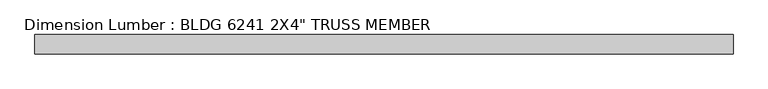
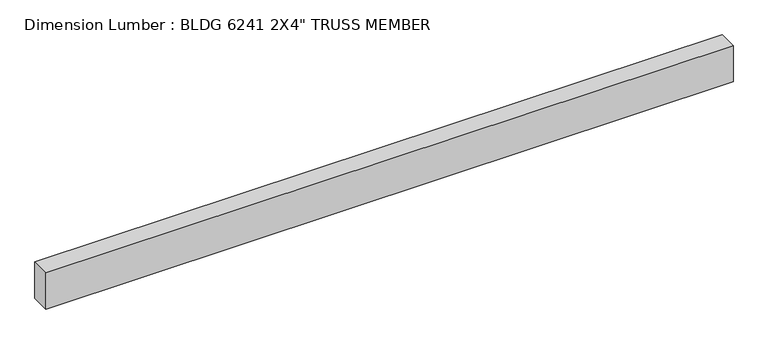
"""IFC4 building model written with IfcOpenShell, lengths in millimetres: beam geometry."""

import ifcopenshell
import ifcopenshell.guid

model = None  # the IFC model being written
_history = None  # IfcOwnerHistory: only IFC2X3 demands one
_inside = {}  # id of a spatial element -> (the spatial element, [elements in it])
_under = {}  # id of a project, library or spatial element -> (it, [spatial elements below it])
_declared = {}  # id of a project -> (the project, [libraries it declares])
_typed = {}  # id of a type object -> (the type object, [elements of that type])
_made_of = {}  # id of a material, layer set ... -> (it, [elements and type objects made of it])


def new_model(schema):
    """Start an empty IFC model of exactly this schema.

    Asked for "IFC4X3", IfcOpenShell would pick the latest addendum, in which some entities
    have other attributes; the version numbers below select the first issue.
    IFC2X3 requires an IfcOwnerHistory on every rooted entity: one is made here for all.
    """
    global model, _history
    if schema == "IFC4X3":
        model = ifcopenshell.file(schema_version=(4, 3, 0, 0))
    else:
        model = ifcopenshell.file(schema=schema)
    _inside.clear()
    _under.clear()
    _declared.clear()
    _typed.clear()
    _made_of.clear()
    _history = None
    if model.schema == "IFC2X3":
        org = make("IfcOrganization", Name="unknown")
        user = make(
            "IfcPersonAndOrganization",
            ThePerson=make("IfcPerson", FamilyName="unknown"),
            TheOrganization=org,
        )
        app = make(
            "IfcApplication",
            ApplicationDeveloper=org,
            Version="unknown",
            ApplicationFullName="unknown",
            ApplicationIdentifier="unknown",
        )
        _history = make(
            "IfcOwnerHistory",
            OwningUser=user,
            OwningApplication=app,
            ChangeAction="ADDED",
            CreationDate=0,
        )
    return model


def make(cls, **values):
    """One entity of the class cls with the attributes given. An attribute that is None is left unset."""
    return model.create_entity(
        cls, **{name: value for name, value in values.items() if value is not None}
    )


def rooted(cls, **values):
    """An entity with a GlobalId (a new one), such as an element, a storey or a relation."""
    return make(cls, GlobalId=ifcopenshell.guid.new(), OwnerHistory=_history, **values)


def si_unit(unit_type, name, prefix=None):
    """IfcSIUnit, for example si_unit("LENGTHUNIT", "METRE", prefix="MILLI")."""
    return make("IfcSIUnit", UnitType=unit_type, Prefix=prefix, Name=name)


def assignment(units):
    """IfcUnitAssignment: the units of a project."""
    return None if units is None else make("IfcUnitAssignment", Units=units)


def point(xyz):
    """IfcCartesianPoint."""
    return None if xyz is None else make("IfcCartesianPoint", Coordinates=xyz)


def direction(xyz):
    """IfcDirection."""
    return None if xyz is None else make("IfcDirection", DirectionRatios=xyz)


def frame(location, z_axis=None, x_axis=None):
    """IfcAxis2Placement3D, a coordinate frame: its origin and axes. An axis left out is left unset."""
    return make(
        "IfcAxis2Placement3D",
        Location=point(location),
        Axis=direction(z_axis),
        RefDirection=direction(x_axis),
    )


def origin():
    """The frame at (0, 0, 0) with its axes left unset."""
    return frame((0.0, 0.0, 0.0))


def place(relative_to, where):
    """IfcLocalPlacement: puts the frame where relative to a parent placement (None: the world)."""
    return make(
        "IfcLocalPlacement", PlacementRelTo=relative_to, RelativePlacement=where
    )


def context(
    kind, dimensions, precision=None, world=None, true_north=None, identifier=None
):
    """IfcGeometricRepresentationContext, for example the 3D "Model" context."""
    return make(
        "IfcGeometricRepresentationContext",
        ContextIdentifier=identifier,
        ContextType=kind,
        CoordinateSpaceDimension=dimensions,
        Precision=precision,
        WorldCoordinateSystem=world,
        TrueNorth=true_north,
    )


def project(units=None, contexts=None):
    """IfcProject with its units and contexts."""
    return rooted(
        "IfcProject",
        Name="project",
        RepresentationContexts=contexts,
        UnitsInContext=assignment(units),
    )


def spatial(cls, under=None, at=None, **own):
    """A site, building, storey or space (cls), placed at a placement, below another one or the project."""
    s = rooted(cls, ObjectPlacement=at, **own)
    if under is not None:
        _under.setdefault(under.id(), (under, []))[1].append(s)
    return s


def polyline(points):
    """IfcPolyline through the points."""
    return make("IfcPolyline", Points=[point(p) for p in points])


def outline(outer, holes=None, kind="AREA"):
    """IfcArbitraryClosedProfileDef: a profile drawn as a closed curve; with holes, ...WithVoids."""
    if holes is None:
        return make("IfcArbitraryClosedProfileDef", ProfileType=kind, OuterCurve=outer)
    return make(
        "IfcArbitraryProfileDefWithVoids",
        ProfileType=kind,
        OuterCurve=outer,
        InnerCurves=holes,
    )


def extrude(swept, where, along, depth):
    """IfcExtrudedAreaSolid: the profile swept, set in the frame where, extruded along a direction by depth."""
    return make(
        "IfcExtrudedAreaSolid",
        SweptArea=swept,
        Position=where,
        ExtrudedDirection=direction(along),
        Depth=depth,
    )


def shape(context_of_items, identifier, shape_type, items):
    """IfcShapeRepresentation: the items that make up one representation, for example the "Body"."""
    return make(
        "IfcShapeRepresentation",
        ContextOfItems=context_of_items,
        RepresentationIdentifier=identifier,
        RepresentationType=shape_type,
        Items=items,
    )


def source(mapping_origin, context_of_items, identifier, shape_type, items):
    """IfcRepresentationMap: a shape defined once, which mapped items show again and again."""
    return make(
        "IfcRepresentationMap",
        MappingOrigin=mapping_origin,
        MappedRepresentation=shape(context_of_items, identifier, shape_type, items),
    )


def transform(
    local_origin,
    x_axis=None,
    y_axis=None,
    z_axis=None,
    scale=None,
    scale2=None,
    scale3=None,
    uniform=True,
):
    """IfcCartesianTransformationOperator3D, or its non-uniform kind. x_axis, y_axis, z_axis: its Axis1, 2, 3."""
    if uniform:
        return make(
            "IfcCartesianTransformationOperator3D",
            Axis1=direction(x_axis),
            Axis2=direction(y_axis),
            LocalOrigin=point(local_origin),
            Scale=scale,
            Axis3=direction(z_axis),
        )
    return make(
        "IfcCartesianTransformationOperator3DnonUniform",
        Axis1=direction(x_axis),
        Axis2=direction(y_axis),
        LocalOrigin=point(local_origin),
        Scale=scale,
        Axis3=direction(z_axis),
        Scale2=scale2,
        Scale3=scale3,
    )


def mapped(mapping_source, mapping_target):
    """IfcMappedItem: shows the shape of a source again, moved by a transform."""
    return make(
        "IfcMappedItem", MappingSource=mapping_source, MappingTarget=mapping_target
    )


def made_of(thing, what):
    """Note that an element or type object is made of a material, layer set ...; save() writes the relation."""
    if what is not None:
        _made_of.setdefault(what.id(), (what, []))[1].append(thing)
    return thing


def element(
    cls,
    number,
    at=None,
    inside=None,
    cuts=None,
    type_object=None,
    material=None,
    context=None,
    identifier="Body",
    shape_type=None,
    held_by="IfcProductDefinitionShape",
    body=None,
    shapes=None,
    **own,
):
    """One element of the class cls, such as IfcWall. Its Tag is "e" and its number.

    at: its placement. inside: the storey or other place that contains it. cuts: it is an
    opening in that element (IfcRelVoidsElement). A single representation is given by context,
    identifier, shape_type and body (its items); several are given by shapes. held_by: the class
    of the entity that holds the representations. save() writes the other relations.
    """
    e = rooted(cls, Tag="e%d" % number, ObjectPlacement=at, **own)
    if body is not None:
        shapes = [shape(context, identifier, shape_type, body)]
    if shapes is not None:
        e.Representation = make(held_by, Representations=shapes)
    if inside is not None:
        _inside.setdefault(inside.id(), (inside, []))[1].append(e)
    if cuts is not None:
        rooted(
            "IfcRelVoidsElement", RelatingBuildingElement=cuts, RelatedOpeningElement=e
        )
    if type_object is not None:
        _typed.setdefault(type_object.id(), (type_object, []))[1].append(e)
    return made_of(e, material)


def aggregate(whole, parts):
    """IfcRelAggregates: a whole, such as a stair, and the parts it consists of."""
    return rooted("IfcRelAggregates", RelatingObject=whole, RelatedObjects=parts)


def save(model, path):
    """Write the relations noted so far, then the file.

    IfcRelAggregates (storeys below a building ...), IfcRelContainedInSpatialStructure (elements
    in a storey), IfcRelDefinesByType, IfcRelAssociatesMaterial and IfcRelDeclares: one each for
    every whole, place, type object, material and project.
    """
    for whole, parts in _under.values():
        aggregate(whole, parts)
    for where, things in _inside.values():
        rooted(
            "IfcRelContainedInSpatialStructure",
            RelatedElements=things,
            RelatingStructure=where,
        )
    for kind, things in _typed.values():
        rooted("IfcRelDefinesByType", RelatedObjects=things, RelatingType=kind)
    for what, things in _made_of.values():
        rooted("IfcRelAssociatesMaterial", RelatedObjects=things, RelatingMaterial=what)
    for by, libraries in _declared.values():
        rooted("IfcRelDeclares", RelatingContext=by, RelatedDefinitions=libraries)
    model.write(path)


def beam_17170791(model_context):
    return source(origin(), model_context, "Body", "SweptSolid", [
        extrude(outline(polyline([(914.3999994, 25.4), (914.3999994, -25.4), (-914.3999994, -25.4), (-914.3999994, 25.4), (914.3999994, 25.4)])), frame((0.0, 0.0, -50.8), z_axis=(0.0, 0.0, 1.0), x_axis=(1.0, 0.0, 0.0)), (0.0, 0.0, 1.0), 101.6),
    ])


if __name__ == "__main__":
    model = new_model("IFC4")
    model_context = context("Model", 3, world=origin())
    ifc_project = project(units=[si_unit("LENGTHUNIT", "METRE", prefix="MILLI")], contexts=[model_context])
    site = spatial("IfcSite", under=ifc_project)
    building = spatial("IfcBuilding", under=site)
    placement = place(None, origin())
    beam_shape = beam_17170791(model_context)
    element("IfcBeam", 1, ObjectType="Dimension Lumber : BLDG 6241 2X4\" TRUSS MEMBER", at=placement, inside=building, context=model_context, shape_type="MappedRepresentation", body=[
        mapped(beam_shape, transform((0.0, 0.0, 0.0), x_axis=(1.0, 0.0, 0.0), y_axis=(0.0, 1.0, 0.0), z_axis=(0.0, 0.0, 1.0))),
    ])
    save(model, "model.ifc")

# Revit data of these elements
# Type "Dimension Lumber : BLDG 6241 2X4\" TRUSS MEMBER"
#   Assembly Code = "B10"
#   A = 0.273472 SF
#   Length [instance default] = 5' - 0"
#   b = 0' - 2"
#   d = 0' - 4"
#   Structural Material [instance default] = Softwood, Lumber
# Element 1 (IfcBeam, "Dimension Lumber : BLDG 6241 2X4\" TRUSS MEMBER")
#   Materials on its faces: "Softwood, Lumber"
# Materials
#   "Softwood, Lumber": class "Wood", colour RGB 223 192 134, transparency 0, Description = "Pinus Echinata", Cost = 0
